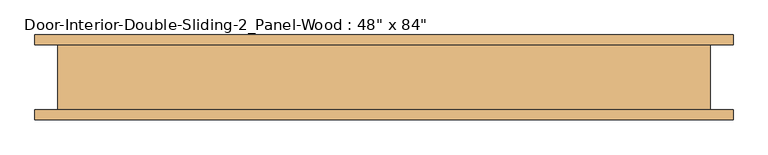
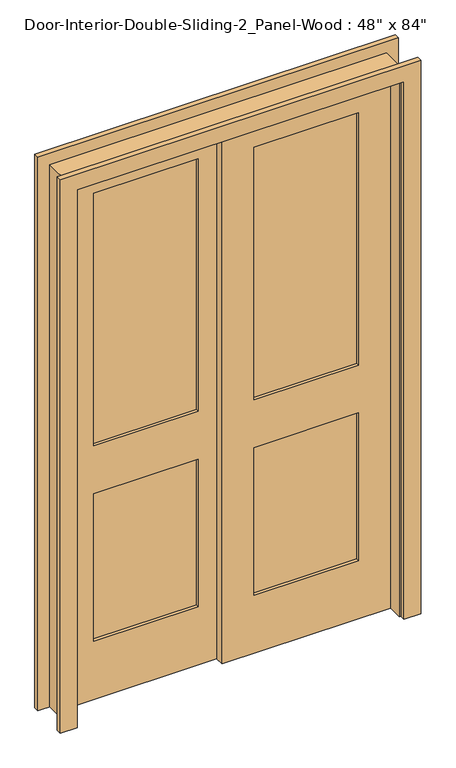
"""IFC4 building model written with IfcOpenShell, lengths in millimetres: door geometry."""

from ifc_helpers import new_model, si_unit, frame, origin, place, context, project, spatial, polyline, outline, extrude, source, transform, mapped, element, save


def door_38ea5fad(model_context):
    return source(origin(), model_context, "Body", "SweptSolid", [
        extrude(outline(polyline([(488.95, 2.1166667), (95.25, 2.1166667), (95.25, 13.7583333), (488.95, 13.7583333), (488.95, 2.1166667)])), frame((0.0, 0.0, 1009.65), z_axis=(0.0, 0.0, 1.0), x_axis=(1.0, 0.0, 0.0)), (0.0, 0.0, 1.0), 1004.8875),
        extrude(outline(polyline([(488.95, 2.1166667), (95.25, 2.1166667), (95.25, 13.7583333), (488.95, 13.7583333), (488.95, 2.1166667)])), frame((0.0, 0.0, 231.775), z_axis=(0.0, 0.0, 1.0), x_axis=(1.0, 0.0, 0.0)), (0.0, 0.0, 1.0), 587.375),
        extrude(outline(polyline([(2133.6, -25.4), (0.0, -25.4), (0.0, 609.6), (2133.6, 609.6), (2133.6, -25.4)]), holes=[polyline([(2014.5375, 95.25), (2014.5375, 488.95), (1009.65, 488.95), (1009.65, 95.25), (2014.5375, 95.25)]), polyline([(819.15, 95.25), (819.15, 488.95), (231.775, 488.95), (231.775, 95.25), (819.15, 95.25)])]), frame((0.0, -9.525, 0.0), z_axis=(0.0, 1.0, 0.0), x_axis=(0.0, 0.0, 1.0)), (0.0, 0.0, 1.0), 34.925),
        extrude(outline(polyline([(-95.25, 37.0416667), (-488.95, 37.0416667), (-488.95, 48.6833333), (-95.25, 48.6833333), (-95.25, 37.0416667)])), frame((0.0, 0.0, 1009.65), z_axis=(0.0, 0.0, 1.0), x_axis=(1.0, 0.0, 0.0)), (0.0, 0.0, 1.0), 1004.8875),
        extrude(outline(polyline([(-95.25, 37.0416667), (-488.95, 37.0416667), (-488.95, 48.6833333), (-95.25, 48.6833333), (-95.25, 37.0416667)])), frame((0.0, 0.0, 231.775), z_axis=(0.0, 0.0, 1.0), x_axis=(1.0, 0.0, 0.0)), (0.0, 0.0, 1.0), 587.375),
        extrude(outline(polyline([(2133.6, -609.6), (0.0, -609.6), (0.0, 25.4), (2133.6, 25.4), (2133.6, -609.6)]), holes=[polyline([(2014.5375, -488.95), (2014.5375, -95.25), (1009.65, -95.25), (1009.65, -488.95), (2014.5375, -488.95)]), polyline([(819.15, -488.95), (819.15, -95.25), (231.775, -95.25), (231.775, -488.95), (819.15, -488.95)])]), frame((0.0, 25.4, 0.0), z_axis=(0.0, 1.0, 0.0), x_axis=(0.0, 0.0, 1.0)), (0.0, 0.0, 1.0), 34.925),
        extrude(outline(polyline([(0.0, 609.6), (0.0, 635.0), (2159.0, 635.0), (2159.0, -635.0), (0.0, -635.0), (0.0, -609.6), (2133.6, -609.6), (2133.6, 609.6), (0.0, 609.6)])), frame((0.0, -66.675, 0.0), z_axis=(0.0, 1.0, 0.0), x_axis=(0.0, 0.0, 1.0)), (0.0, 0.0, 1.0), 127.0),
        extrude(outline(polyline([(0.0, 615.95), (0.0, 679.45), (2203.45, 679.45), (2203.45, -679.45), (0.0, -679.45), (0.0, -615.95), (2139.95, -615.95), (2139.95, 615.95), (0.0, 615.95)])), frame((0.0, -85.725, 0.0), z_axis=(0.0, 1.0, 0.0), x_axis=(0.0, 0.0, 1.0)), (0.0, 0.0, 1.0), 19.05),
        extrude(outline(polyline([(0.0, 615.95), (0.0, 679.45), (2203.45, 679.45), (2203.45, -679.45), (0.0, -679.45), (0.0, -615.95), (2139.95, -615.95), (2139.95, 615.95), (0.0, 615.95)])), frame((0.0, 60.325, 0.0), z_axis=(0.0, 1.0, 0.0), x_axis=(0.0, 0.0, 1.0)), (0.0, 0.0, 1.0), 19.05),
    ])


if __name__ == "__main__":
    model = new_model("IFC4")
    model_context = context("Model", 3, world=origin())
    ifc_project = project(units=[si_unit("LENGTHUNIT", "METRE", prefix="MILLI")], contexts=[model_context])
    site = spatial("IfcSite", under=ifc_project)
    building = spatial("IfcBuilding", under=site)
    placement = place(None, origin())
    door_shape = door_38ea5fad(model_context)
    element("IfcDoor", 1, ObjectType="Door-Interior-Double-Sliding-2_Panel-Wood : 48\" x 84\"", at=placement, inside=building, context=model_context, shape_type="MappedRepresentation", body=[
        mapped(door_shape, transform((0.0, 0.0, 0.0), x_axis=(1.0, 0.0, 0.0), y_axis=(0.0, 1.0, 0.0), z_axis=(0.0, 0.0, 1.0))),
    ])
    save(model, "model.ifc")

# Revit data of these elements
# Type "Door-Interior-Double-Sliding-2_Panel-Wood : 48\" x 84\""
#   Type Mark = "13"
#   Assembly Code = "C1020300"
#   Analytic Construction = "Wooden"
#   Top Rail = 0' - 4 11/16"
#   Thickness = 0' - 1 3/8"
#   Thermal Resistance (R) = 2.5876 (h·ft²·°F)/BTU
#   Stiles = 0' - 4 3/4"
#   Rough Width = 4' - 2"
#   Rough Height = 7' - 1"
#   Lock Rail = 0' - 7 1/2"
#   Height = 7' - 0"
#   Width = 4' - 0"
#   Heat Transfer Coefficient (U) = 0.3865 BTU/(h·ft²·°F)
#   Bottom Rail = 0' - 9 1/8"
#   Function = 0
#   Define Thermal Properties by = 1
#   Trim Material = Cherry
#   Panel Material = Cherry
#   Frame Material = Cherry
#   Visual Light Transmittance = 0
#   Solar Heat Gain Coefficient = 0
#   Wall Closure = (empty or 0)
#   Function = (empty or 0)
# Element 1 (IfcDoor, "Door-Interior-Double-Sliding-2_Panel-Wood : 48\" x 84\"")
#   Materials on its faces: "Cherry"
# Materials
#   "Cherry": class "Wood", colour RGB 157 77 38, transparency 0, Description = "Prunus Serotina", Cost = 0
